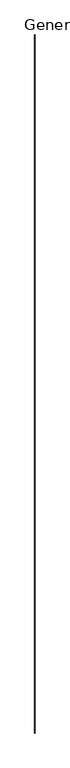
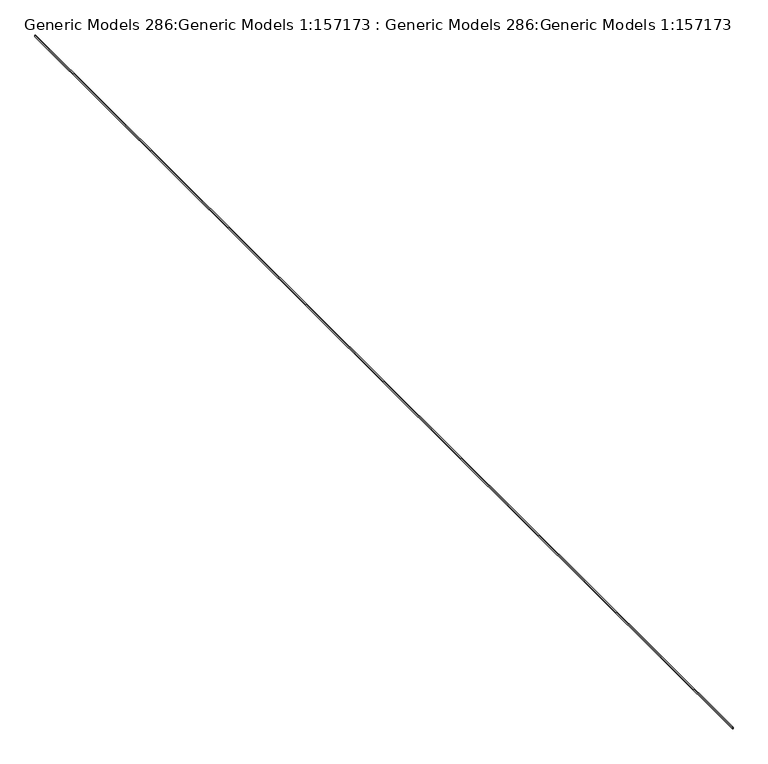
"""IFC4 building model written with IfcOpenShell, lengths in millimetres: proxy geometry, Generic Models 286:Generic Models 1:157173 : Generic Models 286:Generic Models 1:157173."""

from ifc_helpers import new_model, si_unit, point, frame, frame_2d, origin, place, context, project, spatial, polyline, circle_curve, trimmed, segment, composite_curve, outline, extrude, source, transform, mapped, element, save


def generic_models_286_generic_models_1_157173_generic_models_c62aeef5(model_context):
    return source(origin(), model_context, "Body", "SweptSolid", [
        extrude(outline(composite_curve([segment(trimmed(circle_curve(frame_2d((6211.8958727, 1417.0202178)), 4.3100275), [point((6214.8106132, 1420.1952178))], [point((6214.8106132, 1413.8452178))], False, "CARTESIAN"), True, "CONTINUOUS"), segment(polyline([(6214.8106132, 1413.8452178), (6205.2856132, 1413.8452178)]), True, "CONTINUOUS"), segment(trimmed(circle_curve(frame_2d((6202.3708727, 1417.0202178)), 4.3100275), [point((6205.2856132, 1413.8452178))], [point((6205.2856132, 1420.1952178))], True, "CARTESIAN"), True, "CONTINUOUS"), segment(polyline([(6205.2856132, 1420.1952178), (6214.8106132, 1420.1952178)]), True, "CONTINUOUS")], self_intersect=False)), frame((0.0, 496.8218843, 0.0), z_axis=(0.0, 1.0, 0.0), x_axis=(0.0, 0.0, 1.0)), (0.0, 0.0, 1.0), 7886.7),
    ])


if __name__ == "__main__":
    model = new_model("IFC4")
    model_context = context("Model", 3, world=origin())
    ifc_project = project(units=[si_unit("LENGTHUNIT", "METRE", prefix="MILLI")], contexts=[model_context])
    site = spatial("IfcSite", under=ifc_project)
    building = spatial("IfcBuilding", under=site)
    placement = place(None, origin())
    generic_models_286_generic_models_1_157173_generic_models_shape = generic_models_286_generic_models_1_157173_generic_models_c62aeef5(model_context)
    element("IfcBuildingElementProxy", 1, Name="Generic Models 286:Generic Models 1:157173 : Generic Models 286:Generic Models 1:157173", ObjectType="Generic Models 286:Generic Models 1:157173 : Generic Models 286:Generic Models 1:157173", at=placement, inside=building, context=model_context, shape_type="MappedRepresentation", body=[
        mapped(generic_models_286_generic_models_1_157173_generic_models_shape, transform((0.0, 0.0, 0.0), x_axis=(1.0, 0.0, 0.0), y_axis=(0.0, 1.0, 0.0), z_axis=(0.0, 0.0, 1.0))),
    ])
    save(model, "model.ifc")

# Revit data of these elements
# Type "Generic Models 286:Generic Models 1:157173 : Generic Models 286:Generic Models 1:157173"
#   NameOverride = "Generic Models 286:Generic Models 1:157173"
#   ObjectTypeOverride = "Generic Models 286:Generic Models 1"
#   Reference = "Generic Models 1"
#   Category = "Generic Models"
#   Tag = "157173"
# Element 1 (IfcBuildingElementProxy, "Generic Models 286:Generic Models 1:157173 : Generic Models 286:Generic Models 1:157173")
#   Materials on its faces: "_SEALANT JOINT 27113"
# Materials
#   "_SEALANT JOINT 27113": class "Unassigned", colour RGB 190 220 196, transparency 0
